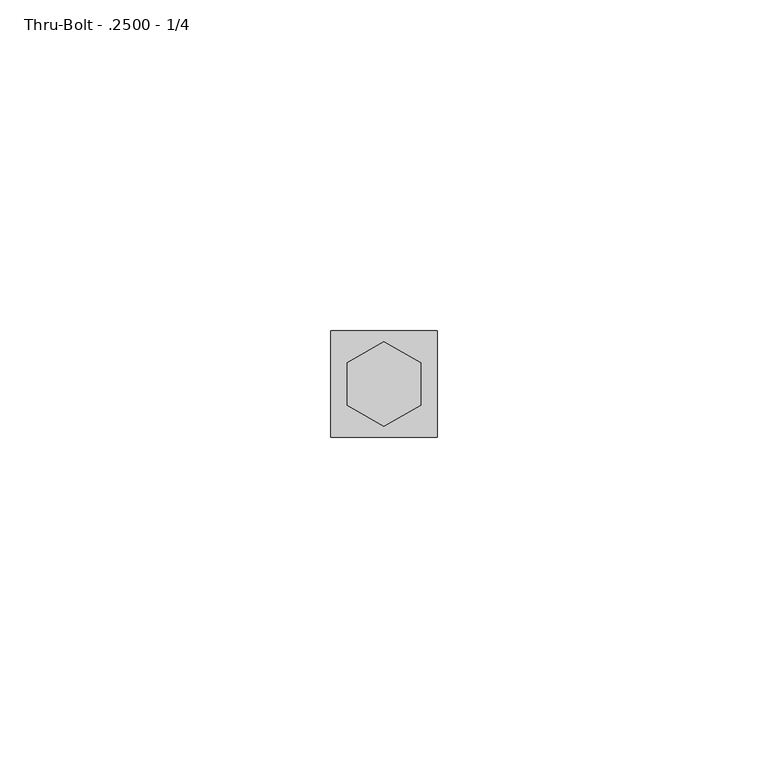
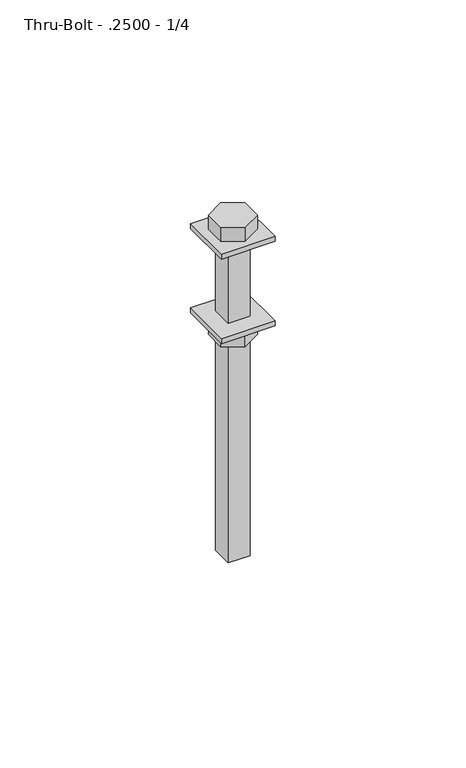
"""IFC4 building model written with IfcOpenShell, lengths in millimetres: fastener geometry, 060523 - W_P_C - Fastenings - Generic - SQUARE : Thru-Bolt - .2500 - 1/4."""

import ifcopenshell
import ifcopenshell.guid

model = None  # the IFC model being written
_history = None  # IfcOwnerHistory: only IFC2X3 demands one
_inside = {}  # id of a spatial element -> (the spatial element, [elements in it])
_under = {}  # id of a project, library or spatial element -> (it, [spatial elements below it])
_declared = {}  # id of a project -> (the project, [libraries it declares])
_typed = {}  # id of a type object -> (the type object, [elements of that type])
_made_of = {}  # id of a material, layer set ... -> (it, [elements and type objects made of it])


def new_model(schema):
    """Start an empty IFC model of exactly this schema.

    Asked for "IFC4X3", IfcOpenShell would pick the latest addendum, in which some entities
    have other attributes; the version numbers below select the first issue.
    IFC2X3 requires an IfcOwnerHistory on every rooted entity: one is made here for all.
    """
    global model, _history
    if schema == "IFC4X3":
        model = ifcopenshell.file(schema_version=(4, 3, 0, 0))
    else:
        model = ifcopenshell.file(schema=schema)
    _inside.clear()
    _under.clear()
    _declared.clear()
    _typed.clear()
    _made_of.clear()
    _history = None
    if model.schema == "IFC2X3":
        org = make("IfcOrganization", Name="unknown")
        user = make(
            "IfcPersonAndOrganization",
            ThePerson=make("IfcPerson", FamilyName="unknown"),
            TheOrganization=org,
        )
        app = make(
            "IfcApplication",
            ApplicationDeveloper=org,
            Version="unknown",
            ApplicationFullName="unknown",
            ApplicationIdentifier="unknown",
        )
        _history = make(
            "IfcOwnerHistory",
            OwningUser=user,
            OwningApplication=app,
            ChangeAction="ADDED",
            CreationDate=0,
        )
    return model


def make(cls, **values):
    """One entity of the class cls with the attributes given. An attribute that is None is left unset."""
    return model.create_entity(
        cls, **{name: value for name, value in values.items() if value is not None}
    )


def rooted(cls, **values):
    """An entity with a GlobalId (a new one), such as an element, a storey or a relation."""
    return make(cls, GlobalId=ifcopenshell.guid.new(), OwnerHistory=_history, **values)


def si_unit(unit_type, name, prefix=None):
    """IfcSIUnit, for example si_unit("LENGTHUNIT", "METRE", prefix="MILLI")."""
    return make("IfcSIUnit", UnitType=unit_type, Prefix=prefix, Name=name)


def assignment(units):
    """IfcUnitAssignment: the units of a project."""
    return None if units is None else make("IfcUnitAssignment", Units=units)


def point(xyz):
    """IfcCartesianPoint."""
    return None if xyz is None else make("IfcCartesianPoint", Coordinates=xyz)


def direction(xyz):
    """IfcDirection."""
    return None if xyz is None else make("IfcDirection", DirectionRatios=xyz)


def frame(location, z_axis=None, x_axis=None):
    """IfcAxis2Placement3D, a coordinate frame: its origin and axes. An axis left out is left unset."""
    return make(
        "IfcAxis2Placement3D",
        Location=point(location),
        Axis=direction(z_axis),
        RefDirection=direction(x_axis),
    )


def origin():
    """The frame at (0, 0, 0) with its axes left unset."""
    return frame((0.0, 0.0, 0.0))


def origin_with_axes():
    """The frame at (0, 0, 0) with the z axis (0, 0, 1) and the x axis (1, 0, 0) written out."""
    return frame((0.0, 0.0, 0.0), z_axis=(0.0, 0.0, 1.0), x_axis=(1.0, 0.0, 0.0))


def place(relative_to, where):
    """IfcLocalPlacement: puts the frame where relative to a parent placement (None: the world)."""
    return make(
        "IfcLocalPlacement", PlacementRelTo=relative_to, RelativePlacement=where
    )


def context(
    kind, dimensions, precision=None, world=None, true_north=None, identifier=None
):
    """IfcGeometricRepresentationContext, for example the 3D "Model" context."""
    return make(
        "IfcGeometricRepresentationContext",
        ContextIdentifier=identifier,
        ContextType=kind,
        CoordinateSpaceDimension=dimensions,
        Precision=precision,
        WorldCoordinateSystem=world,
        TrueNorth=true_north,
    )


def project(units=None, contexts=None):
    """IfcProject with its units and contexts."""
    return rooted(
        "IfcProject",
        Name="project",
        RepresentationContexts=contexts,
        UnitsInContext=assignment(units),
    )


def spatial(cls, under=None, at=None, **own):
    """A site, building, storey or space (cls), placed at a placement, below another one or the project."""
    s = rooted(cls, ObjectPlacement=at, **own)
    if under is not None:
        _under.setdefault(under.id(), (under, []))[1].append(s)
    return s


def polyline(points):
    """IfcPolyline through the points."""
    return make("IfcPolyline", Points=[point(p) for p in points])


def outline(outer, holes=None, kind="AREA"):
    """IfcArbitraryClosedProfileDef: a profile drawn as a closed curve; with holes, ...WithVoids."""
    if holes is None:
        return make("IfcArbitraryClosedProfileDef", ProfileType=kind, OuterCurve=outer)
    return make(
        "IfcArbitraryProfileDefWithVoids",
        ProfileType=kind,
        OuterCurve=outer,
        InnerCurves=holes,
    )


def extrude(swept, where, along, depth):
    """IfcExtrudedAreaSolid: the profile swept, set in the frame where, extruded along a direction by depth."""
    return make(
        "IfcExtrudedAreaSolid",
        SweptArea=swept,
        Position=where,
        ExtrudedDirection=direction(along),
        Depth=depth,
    )


def shape(context_of_items, identifier, shape_type, items):
    """IfcShapeRepresentation: the items that make up one representation, for example the "Body"."""
    return make(
        "IfcShapeRepresentation",
        ContextOfItems=context_of_items,
        RepresentationIdentifier=identifier,
        RepresentationType=shape_type,
        Items=items,
    )


def source(mapping_origin, context_of_items, identifier, shape_type, items):
    """IfcRepresentationMap: a shape defined once, which mapped items show again and again."""
    return make(
        "IfcRepresentationMap",
        MappingOrigin=mapping_origin,
        MappedRepresentation=shape(context_of_items, identifier, shape_type, items),
    )


def transform(
    local_origin,
    x_axis=None,
    y_axis=None,
    z_axis=None,
    scale=None,
    scale2=None,
    scale3=None,
    uniform=True,
):
    """IfcCartesianTransformationOperator3D, or its non-uniform kind. x_axis, y_axis, z_axis: its Axis1, 2, 3."""
    if uniform:
        return make(
            "IfcCartesianTransformationOperator3D",
            Axis1=direction(x_axis),
            Axis2=direction(y_axis),
            LocalOrigin=point(local_origin),
            Scale=scale,
            Axis3=direction(z_axis),
        )
    return make(
        "IfcCartesianTransformationOperator3DnonUniform",
        Axis1=direction(x_axis),
        Axis2=direction(y_axis),
        LocalOrigin=point(local_origin),
        Scale=scale,
        Axis3=direction(z_axis),
        Scale2=scale2,
        Scale3=scale3,
    )


def mapped(mapping_source, mapping_target):
    """IfcMappedItem: shows the shape of a source again, moved by a transform."""
    return make(
        "IfcMappedItem", MappingSource=mapping_source, MappingTarget=mapping_target
    )


def made_of(thing, what):
    """Note that an element or type object is made of a material, layer set ...; save() writes the relation."""
    if what is not None:
        _made_of.setdefault(what.id(), (what, []))[1].append(thing)
    return thing


def element(
    cls,
    number,
    at=None,
    inside=None,
    cuts=None,
    type_object=None,
    material=None,
    context=None,
    identifier="Body",
    shape_type=None,
    held_by="IfcProductDefinitionShape",
    body=None,
    shapes=None,
    **own,
):
    """One element of the class cls, such as IfcWall. Its Tag is "e" and its number.

    at: its placement. inside: the storey or other place that contains it. cuts: it is an
    opening in that element (IfcRelVoidsElement). A single representation is given by context,
    identifier, shape_type and body (its items); several are given by shapes. held_by: the class
    of the entity that holds the representations. save() writes the other relations.
    """
    e = rooted(cls, Tag="e%d" % number, ObjectPlacement=at, **own)
    if body is not None:
        shapes = [shape(context, identifier, shape_type, body)]
    if shapes is not None:
        e.Representation = make(held_by, Representations=shapes)
    if inside is not None:
        _inside.setdefault(inside.id(), (inside, []))[1].append(e)
    if cuts is not None:
        rooted(
            "IfcRelVoidsElement", RelatingBuildingElement=cuts, RelatedOpeningElement=e
        )
    if type_object is not None:
        _typed.setdefault(type_object.id(), (type_object, []))[1].append(e)
    return made_of(e, material)


def aggregate(whole, parts):
    """IfcRelAggregates: a whole, such as a stair, and the parts it consists of."""
    return rooted("IfcRelAggregates", RelatingObject=whole, RelatedObjects=parts)


def save(model, path):
    """Write the relations noted so far, then the file.

    IfcRelAggregates (storeys below a building ...), IfcRelContainedInSpatialStructure (elements
    in a storey), IfcRelDefinesByType, IfcRelAssociatesMaterial and IfcRelDeclares: one each for
    every whole, place, type object, material and project.
    """
    for whole, parts in _under.values():
        aggregate(whole, parts)
    for where, things in _inside.values():
        rooted(
            "IfcRelContainedInSpatialStructure",
            RelatedElements=things,
            RelatingStructure=where,
        )
    for kind, things in _typed.values():
        rooted("IfcRelDefinesByType", RelatedObjects=things, RelatingType=kind)
    for what, things in _made_of.values():
        rooted("IfcRelAssociatesMaterial", RelatedObjects=things, RelatingMaterial=what)
    for by, libraries in _declared.values():
        rooted("IfcRelDeclares", RelatingContext=by, RelatedDefinitions=libraries)
    model.write(path)


def thru_bolt_2500_1_4_f6ebfea6(model_context):
    return source(origin(), model_context, "Body", "SweptSolid", [
        extrude(outline(polyline([(-8.0645, -8.0645), (-8.0645, 8.0645), (8.0645, 8.0645), (8.0645, -8.0645), (-8.0645, -8.0645)])), origin_with_axes(), (0.0, 0.0, 1.0), 1.5875),
        extrude(outline(polyline([(-8.0645, -8.0645), (-8.0645, 8.0645), (8.0645, 8.0645), (8.0645, -8.0645), (-8.0645, -8.0645)])), frame((0.0, 0.0, -26.9875), z_axis=(0.0, 0.0, 1.0), x_axis=(1.0, 0.0, 0.0)), (0.0, 0.0, 1.0), 1.5875),
        extrude(outline(polyline([(-5.55625, -3.2079024), (-5.55625, 3.2079024), (0.0, 6.4158049), (5.55625, 3.2079024), (5.55625, -3.2079024), (0.0, -6.4158049), (-5.55625, -3.2079024)])), frame((0.0, 0.0, -31.75), z_axis=(0.0, 0.0, 1.0), x_axis=(1.0, 0.0, 0.0)), (0.0, 0.0, 1.0), 4.7625),
        extrude(outline(polyline([(-5.55625, 3.2079024), (0.0, 6.4158049), (5.55625, 3.2079024), (5.55625, -3.2079024), (0.0, -6.4158049), (-5.55625, -3.2079024), (-5.55625, 3.2079024)])), frame((0.0, 0.0, 1.5875), z_axis=(0.0, 0.0, 1.0), x_axis=(1.0, 0.0, 0.0)), (0.0, 0.0, 1.0), 4.7625),
        extrude(outline(polyline([(-3.302, 3.302), (3.302, 3.302), (3.302, -3.302), (-3.302, -3.302), (-3.302, 3.302)])), frame((0.0, 0.0, -101.6), z_axis=(0.0, 0.0, 1.0), x_axis=(1.0, 0.0, 0.0)), (0.0, 0.0, 1.0), 103.1875),
    ])


if __name__ == "__main__":
    model = new_model("IFC4")
    model_context = context("Model", 3, world=origin())
    ifc_project = project(units=[si_unit("LENGTHUNIT", "METRE", prefix="MILLI")], contexts=[model_context])
    site = spatial("IfcSite", under=ifc_project)
    building = spatial("IfcBuilding", under=site)
    placement = place(None, origin())
    thru_bolt_2500_1_4_shape = thru_bolt_2500_1_4_f6ebfea6(model_context)
    element("IfcFastener", 1, ObjectType="060523 - W_P_C - Fastenings - Generic - SQUARE : Thru-Bolt - .2500 - 1/4", at=placement, inside=building, context=model_context, shape_type="MappedRepresentation", body=[
        mapped(thru_bolt_2500_1_4_shape, transform((0.0, 0.0, 0.0), x_axis=(1.0, 0.0, 0.0), y_axis=(0.0, 1.0, 0.0), z_axis=(0.0, 0.0, 1.0))),
    ])
    save(model, "model.ifc")

# Revit data of these elements
# Type "060523 - W_P_C - Fastenings - Generic - SQUARE : Thru-Bolt - .2500 - 1/4"
#   Washer_Thickness = 0' - 0 1/16"
#   Washer Radius = 0' - 0.3175"
#   Washer Offset - Head = 0' - 0 1/16"
#   Washer Offset = 0' - 0 1/16"
#   Thickness_of_Substrate [instance default] = 0' - 1"
#   Side = 0' - 0.25293"
#   Radius = 0' - 0.13"
#   Length [instance default] = 0' - 4"
#   Head Size = 0' - 0 7/16"
#   Head Radius = 0' - 0 7/32"
#   Head Height = 0' - 0 3/16"
#   Double Diameter = 0' - 0.52"
#   Diameter = 0' - 0.26"
#   Default Elevation = 4' - 0"
#   Washer_Nut_Visibility = yes
#   Washer_Head_Visibility = yes
#   Round_Head_Visibility = no
#   Point Visibility = no
#   Nut_Visibility = yes
#   Hex_Head_Visiblilty = yes
#   Washer Material = none
#   Bolt Material (Size) = AT SILL - FASTENER AT 24" O.C.
# Element 1 (IfcFastener, "060523 - W_P_C - Fastenings - Generic - SQUARE : Thru-Bolt - .2500 - 1/4")
#   Materials on its faces: "AT SILL - FASTENER AT 24\" O.C."
# Materials
#   "AT SILL - FASTENER AT 24\" O.C.": class "Generic", colour RGB 120 120 120, transparency 0, Cost = 0
